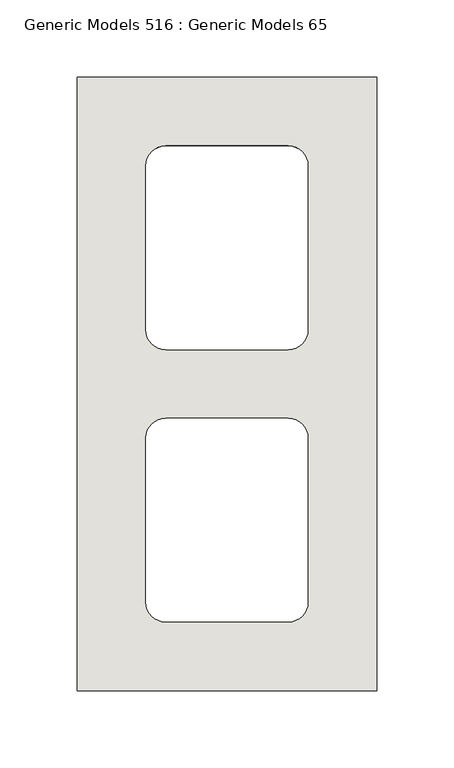
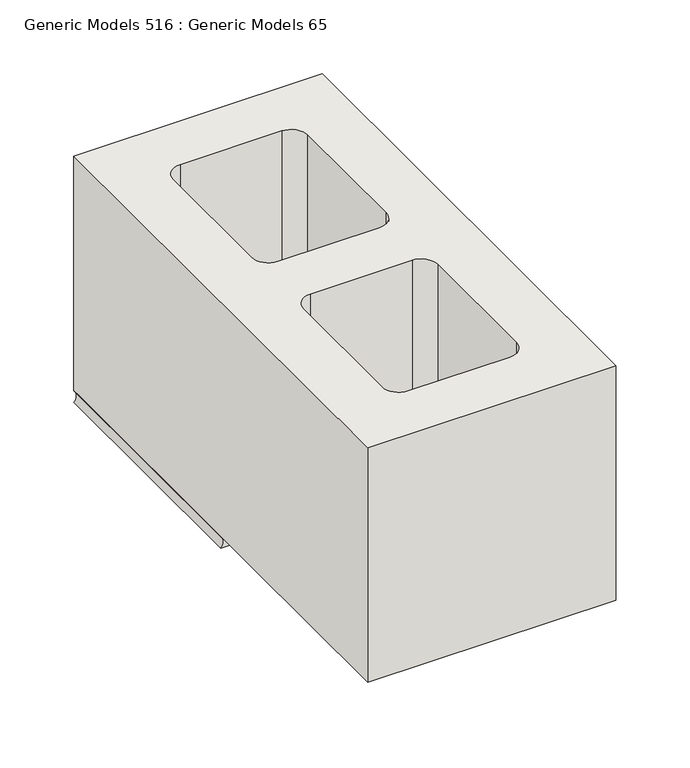
"""IFC4 building model written with IfcOpenShell, lengths in millimetres: wall geometry, Generic Models 516 : Generic Models 65."""

from ifc_helpers import new_model, si_unit, point, frame, frame_2d, origin, place, context, project, spatial, polyline, circle_curve, trimmed, segment, composite_curve, outline, extrude, source, transform, mapped, element, save
from ifc_brep_helpers import plane_surface, revolved_surface, advanced_brep


def generic_models_516_generic_models_65_4e104269(model_context):
    return source(origin(), model_context, "Body", "SolidModel", [
        advanced_brep(
        [(428979.0125, 503.2375, 212.725), (428785.3375, 503.2375, 212.725), (428785.3375, 503.2375, 203.2), (428979.0125, 503.2375, 203.2), (428979.0125, 701.675, 212.725), (428979.0125, 701.675, 203.2), (428785.3375, 701.675, 203.2), (428785.3375, 701.675, 212.725), (428934.5625, 538.1625, 212.725), (428921.8625, 525.4625, 212.725), (428842.4875, 525.4625, 212.725), (428829.7875, 538.1625, 212.725), (428829.7875, 644.525, 212.725), (428842.4875, 657.225, 212.725), (428921.8625, 657.225, 212.725), (428934.5625, 644.525, 212.725), (428921.8625, 525.4625, 203.2), (428934.5625, 538.1625, 203.2), (428842.4875, 525.4625, 203.2), (428829.7875, 538.1625, 203.2), (428829.7875, 644.525, 203.2), (428842.4875, 657.225, 203.2), (428921.8625, 657.225, 203.2), (428934.5625, 644.525, 203.2)],
        [
            (0, 1),
            (1, 2, circle_curve(frame((428780.4545028, 503.2375, 207.9625), z_axis=(0.0, 1.0, 0.0), x_axis=(1.0, 0.0, 0.0)), 6.8209287)),
            (2, 3),
            (3, 0, circle_curve(frame((428983.8954972, 503.2375, 207.9625), z_axis=(0.0, 1.0, 0.0), x_axis=(-1.0, 0.0, 0.0)), 6.8209287)),
            (4, 5, circle_curve(frame((428983.8954972, 701.675, 207.9625), z_axis=(0.0, -1.0, 0.0), x_axis=(-1.0, 0.0, 0.0)), 6.8209287)),
            (5, 6),
            (6, 7, circle_curve(frame((428780.4545028, 701.675, 207.9625), z_axis=(0.0, -1.0, 0.0), x_axis=(1.0, 0.0, 0.0)), 6.8209287)),
            (7, 4),
            (0, 4),
            (7, 1),
            (8, 9, circle_curve(frame((428921.8625, 538.1625, 212.725), z_axis=(0.0, 0.0, -1.0), x_axis=(-1.0, 0.0, 0.0)), 12.7)),
            (9, 10),
            (10, 11, circle_curve(frame((428842.4875, 538.1625, 212.725), z_axis=(0.0, 0.0, -1.0), x_axis=(-1.0, 0.0, 0.0)), 12.7)),
            (11, 12),
            (12, 13, circle_curve(frame((428842.4875, 644.525, 212.725), z_axis=(0.0, 0.0, -1.0), x_axis=(-1.0, 0.0, 0.0)), 12.7)),
            (13, 14),
            (14, 15, circle_curve(frame((428921.8625, 644.525, 212.725), z_axis=(0.0, 0.0, -1.0), x_axis=(-1.0, 0.0, 0.0)), 12.7)),
            (15, 8),
            (16, 9),
            (8, 17),
            (17, 16, circle_curve(frame((428921.8625, 538.1625, 203.2), z_axis=(0.0, 0.0, -1.0), x_axis=(-1.0, 0.0, 0.0)), 12.7)),
            (16, 18),
            (18, 10),
            (18, 19, circle_curve(frame((428842.4875, 538.1625, 203.2), z_axis=(0.0, 0.0, -1.0), x_axis=(-1.0, 0.0, 0.0)), 12.7)),
            (19, 11),
            (19, 20),
            (20, 12),
            (20, 21, circle_curve(frame((428842.4875, 644.525, 203.2), z_axis=(0.0, 0.0, -1.0), x_axis=(-1.0, 0.0, 0.0)), 12.7)),
            (21, 13),
            (21, 22),
            (22, 14),
            (22, 23, circle_curve(frame((428921.8625, 644.525, 203.2), z_axis=(0.0, 0.0, -1.0), x_axis=(-1.0, 0.0, 0.0)), 12.7)),
            (23, 15),
            (23, 17),
            (6, 2),
            (5, 3),
        ],
        [
            plane_surface(frame((428882.175, 503.2375, 213.121875), z_axis=(0.0, -1.0, 0.0), x_axis=(0.0, 0.0, 1.0))),
            plane_surface(frame((428882.175, 701.675, 213.121875), z_axis=(0.0, 1.0, 0.0), x_axis=(0.0, 0.0, 1.0))),
            plane_surface(frame((428979.0125, 503.2375, 212.725), z_axis=(0.0, 0.0, 1.0), x_axis=(0.0, 1.0, 0.0))),
            revolved_surface(polyline([(428909.1625, 538.1625, 212.725), (428909.1625, 538.1625, 203.2)]), (428921.8625, 538.1625, 396.875), (0.0, 0.0, 1.0)),
            plane_surface(frame((428842.4875, 525.4625, 396.875), z_axis=(0.0, 1.0, 0.0), x_axis=(0.0, 0.0, -1.0))),
            revolved_surface(polyline([(428829.7875, 538.1625, 212.725), (428829.7875, 538.1625, 203.2)]), (428842.4875, 538.1625, 396.875), (0.0, 0.0, 1.0)),
            plane_surface(frame((428829.7875, 644.525, 396.875), z_axis=(1.0, 0.0, 0.0), x_axis=(0.0, 0.0, -1.0))),
            revolved_surface(polyline([(428829.7875, 644.525, 212.725), (428829.7875, 644.525, 203.2)]), (428842.4875, 644.525, 396.875), (0.0, 0.0, 1.0)),
            plane_surface(frame((428921.8625, 657.225, 396.875), z_axis=(0.0, -1.0, 0.0), x_axis=(0.0, 0.0, -1.0))),
            revolved_surface(polyline([(428909.1625, 644.525, 212.725), (428909.1625, 644.525, 203.2)]), (428921.8625, 644.525, 396.875), (0.0, 0.0, 1.0)),
            plane_surface(frame((428934.5625, 538.1625, 396.875), z_axis=(-1.0, 0.0, 0.0), x_axis=(0.0, 0.0, -1.0))),
            revolved_surface(polyline([(428787.2754315, 701.675, 207.9625), (428787.2754315, 503.2375, 207.9625)]), (428780.4545028, 503.2375, 207.9625), (0.0, 1.0, 0.0)),
            plane_surface(frame((428785.3375, 503.2375, 203.2), z_axis=(0.0, 0.0, -1.0), x_axis=(0.0, 1.0, 0.0))),
            revolved_surface(polyline([(428977.07456850004, 701.675, 207.9625), (428977.07456850004, 503.2375, 207.9625)]), (428983.8954972, 503.2375, 207.9625), (0.0, 1.0, 0.0)),
        ],
        [
            (0, [[1, 2, 3, 4]]),
            (1, [[5, 6, 7, 8]]),
            (2, [[-1, 9, -8, 10], [11, 12, 13, 14, 15, 16, 17, 18]]),
            (3, [[19, -11, 20, 21]]),
            (4, [[-19, 22, 23, -12]]),
            (5, [[-23, 24, 25, -13]]),
            (6, [[-25, 26, 27, -14]]),
            (7, [[-27, 28, 29, -15]]),
            (8, [[-29, 30, 31, -16]]),
            (9, [[-31, 32, 33, -17]]),
            (10, [[-33, 34, -20, -18]]),
            (11, [[-2, -10, -7, 35]]),
            (12, [[-3, -35, -6, 36], [-21, -34, -32, -30, -28, -26, -24, -22]]),
            (13, [[-4, -36, -5, -9]]),
        ],
    ),
        extrude(outline(polyline([(428979.0125, 304.8), (428785.3375, 304.8), (428785.3375, 701.675), (428979.0125, 701.675), (428979.0125, 304.8)]), holes=[composite_curve([segment(polyline([(428934.5625, 538.1625), (428934.5625, 644.525)]), True, "CONTINUOUS"), segment(trimmed(circle_curve(frame_2d((428921.8625, 644.525)), 12.7), [point((428934.5625, 644.525))], [point((428921.8625, 657.225))], True, "CARTESIAN"), True, "CONTINUOUS"), segment(polyline([(428921.8625, 657.225), (428842.4875, 657.225)]), True, "CONTINUOUS"), segment(trimmed(circle_curve(frame_2d((428842.4875, 644.525)), 12.7), [point((428842.4875, 657.225))], [point((428829.7875, 644.525))], True, "CARTESIAN"), True, "CONTINUOUS"), segment(polyline([(428829.7875, 644.525), (428829.7875, 538.1625)]), True, "CONTINUOUS"), segment(trimmed(circle_curve(frame_2d((428842.4875, 538.1625)), 12.7), [point((428829.7875, 538.1625))], [point((428842.4875, 525.4625))], True, "CARTESIAN"), True, "CONTINUOUS"), segment(polyline([(428842.4875, 525.4625), (428921.8625, 525.4625)]), True, "CONTINUOUS"), segment(trimmed(circle_curve(frame_2d((428921.8625, 538.1625)), 12.7), [point((428921.8625, 525.4625))], [point((428934.5625, 538.1625))], True, "CARTESIAN"), True, "CONTINUOUS")], self_intersect=False), composite_curve([segment(polyline([(428829.7875, 468.3125), (428829.7875, 361.95)]), True, "CONTINUOUS"), segment(trimmed(circle_curve(frame_2d((428842.4875, 361.95)), 12.7), [point((428829.7875, 361.95))], [point((428842.4875, 349.25))], True, "CARTESIAN"), True, "CONTINUOUS"), segment(polyline([(428842.4875, 349.25), (428921.8625, 349.25)]), True, "CONTINUOUS"), segment(trimmed(circle_curve(frame_2d((428921.8625, 361.95)), 12.7), [point((428921.8625, 349.25))], [point((428934.5625, 361.95))], True, "CARTESIAN"), True, "CONTINUOUS"), segment(polyline([(428934.5625, 361.95), (428934.5625, 468.3125)]), True, "CONTINUOUS"), segment(trimmed(circle_curve(frame_2d((428921.8625, 468.3125)), 12.7), [point((428934.5625, 468.3125))], [point((428921.8625, 481.0125))], True, "CARTESIAN"), True, "CONTINUOUS"), segment(polyline([(428921.8625, 481.0125), (428842.4875, 481.0125)]), True, "CONTINUOUS"), segment(trimmed(circle_curve(frame_2d((428842.4875, 468.3125)), 12.7), [point((428842.4875, 481.0125))], [point((428829.7875, 468.3125))], True, "CARTESIAN"), True, "CONTINUOUS")], self_intersect=False)]), frame((0.0, 0.0, 212.725), z_axis=(0.0, 0.0, 1.0), x_axis=(1.0, 0.0, 0.0)), (0.0, 0.0, 1.0), 193.675),
    ])


if __name__ == "__main__":
    model = new_model("IFC4")
    model_context = context("Model", 3, world=origin())
    ifc_project = project(units=[si_unit("LENGTHUNIT", "METRE", prefix="MILLI")], contexts=[model_context])
    site = spatial("IfcSite", under=ifc_project)
    building = spatial("IfcBuilding", under=site)
    placement = place(None, origin())
    generic_models_516_generic_models_65_shape = generic_models_516_generic_models_65_4e104269(model_context)
    element("IfcWall", 1, ObjectType="Generic Models 516 : Generic Models 65", at=placement, inside=building, context=model_context, shape_type="MappedRepresentation", body=[
        mapped(generic_models_516_generic_models_65_shape, transform((0.0, 0.0, 0.0), x_axis=(1.0, 0.0, 0.0), y_axis=(0.0, 1.0, 0.0), z_axis=(0.0, 0.0, 1.0))),
    ])
    save(model, "model.ifc")

# Revit data of these elements
# Element 1 (IfcWall, "Generic Models 516 : Generic Models 65")
#   Materials on its faces: "CMU (SEE 'WALL TAG' FOR SIZE)", "MORTAR JOINT"
# Materials
#   "CMU (SEE 'WALL TAG' FOR SIZE)": class "Masonry", colour RGB 203 203 199, transparency 0, Description = "Concrete masonry units", Cost = 0
#   "MORTAR JOINT": class "Generic", colour RGB 120 120 120, transparency 0, Cost = 0
